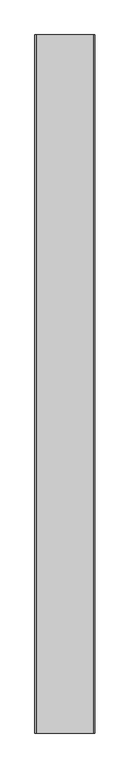
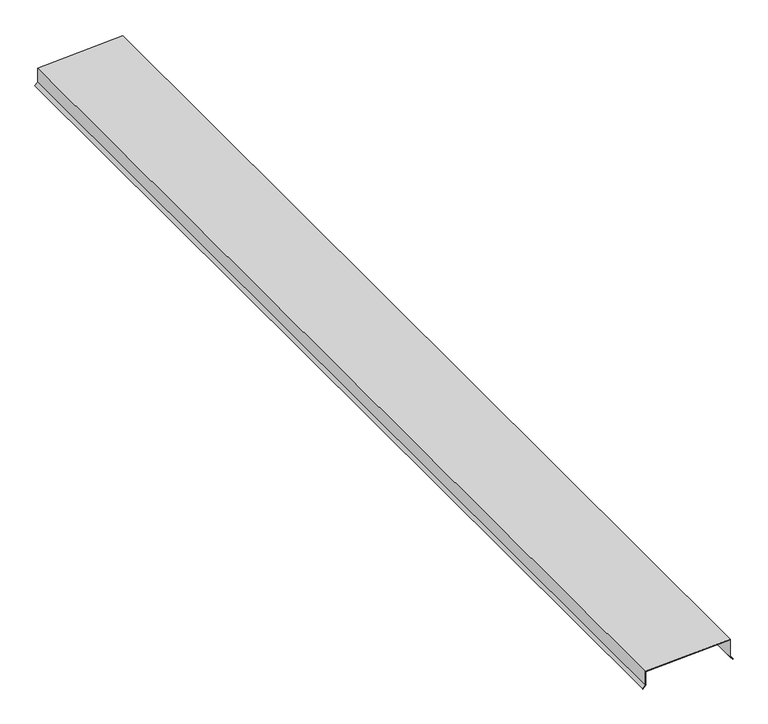
"""IFC4 building model written with IfcOpenShell, lengths in millimetres: proxy geometry, Generic Models 7:Generic Models 1:5:Generic Models 1:5 : Generic Models 7:Generic Models 1:337419:20 : Generic Models 7:Generic Models 1:5:Generic Models 1:5 : Generic Models 7:Generic Models 1:337419:311462."""

from ifc_helpers import new_model, si_unit, frame, origin, place, context, project, spatial, polyline, outline, extrude, source, transform, mapped, element, save


def generic_models_0bbbcb7a(model_context):
    return source(origin(), model_context, "Body", "SweptSolid", [
        extrude(outline(polyline([(6080.7848677, 579480.7492239), (6169.6848677, 579480.7492239), (6149.051925, 579087.0492239), (6080.7848677, 579087.0492239), (6068.0848677, 579074.3492239), (6066.9623357, 579075.4717559), (6080.1273037, 579088.6367239), (6147.5454438, 579088.6367239), (6168.0119918, 579479.1617239), (6080.1273037, 579479.1617239), (6066.9623357, 579492.3266919), (6068.0848677, 579493.4492239), (6080.7848677, 579480.7492239)])), frame((0.0, -572590.3663841, 0.0), z_axis=(0.0, 1.0, 0.0), x_axis=(0.0, 0.0, 1.0)), (0.0, 0.0, 1.0), 4876.8),
    ])


if __name__ == "__main__":
    model = new_model("IFC4")
    model_context = context("Model", 3, world=origin())
    ifc_project = project(units=[si_unit("LENGTHUNIT", "METRE", prefix="MILLI")], contexts=[model_context])
    site = spatial("IfcSite", under=ifc_project)
    building = spatial("IfcBuilding", under=site)
    placement = place(None, origin())
    generic_models_shape = generic_models_0bbbcb7a(model_context)
    element("IfcBuildingElementProxy", 1, Name="Generic Models 7:Generic Models 1:5:Generic Models 1:5 : Generic Models 7:Generic Models 1:337419:20 : Generic Models 7:Generic Models 1:5:Generic Models 1:5 : Generic Models 7:Generic Models 1:337419:311462", ObjectType="Generic Models 7:Generic Models 1:5:Generic Models 1:5 : Generic Models 7:Generic Models 1:337419:20 : Generic Models 7:Generic Models 1:5:Generic Models 1:5 : Generic Models 7:Generic Models 1:337419:311462", at=placement, inside=building, context=model_context, shape_type="MappedRepresentation", body=[
        mapped(generic_models_shape, transform((0.0, 0.0, 0.0), x_axis=(1.0, 0.0, 0.0), y_axis=(0.0, 1.0, 0.0), z_axis=(0.0, 0.0, 1.0))),
    ])
    save(model, "model.ifc")

# Revit data of these elements
# Type "Generic Models 7:Generic Models 1:5:Generic Models 1:5 : Generic Models 7:Generic Models 1:337419:20 : Generic Models 7:Generic Models 1:5:Generic Models 1:5 : Generic Models 7:Generic Models 1:337419:311462"
#   NameOverride = "Generic Models 7:Generic Models 1:5:Generic Models 1:5 : Generic Models 7:Generic Models 1:337419:311462"
#   ObjectTypeOverride = "Generic Models 1:5 : Generic Models 7:Generic Models 1:337419"
#   Reference = "Generic Models 1"
#   Tag = "311462"
# Element 1 (IfcBuildingElementProxy, "Generic Models 7:Generic Models 1:5:Generic Models 1:5 : Generic Models 7:Generic Models 1:337419:20 : Generic Models 7:Generic Models 1:5:Generic Models 1:5 : Generic Models 7:Generic Models 1:337419:311462")
#   Materials on its faces: "SHEET METAL COPING (COLOR TO MATCH RESIN PANEL)"
# Materials
#   "SHEET METAL COPING (COLOR TO MATCH RESIN PANEL)": class "Generic", colour RGB 240 240 240, transparency 0, Keynote = "M07711300.01", Cost = 0
